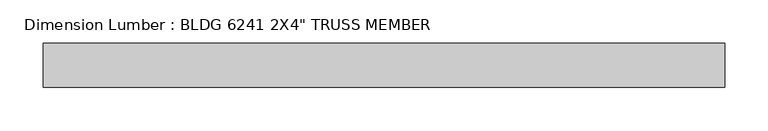
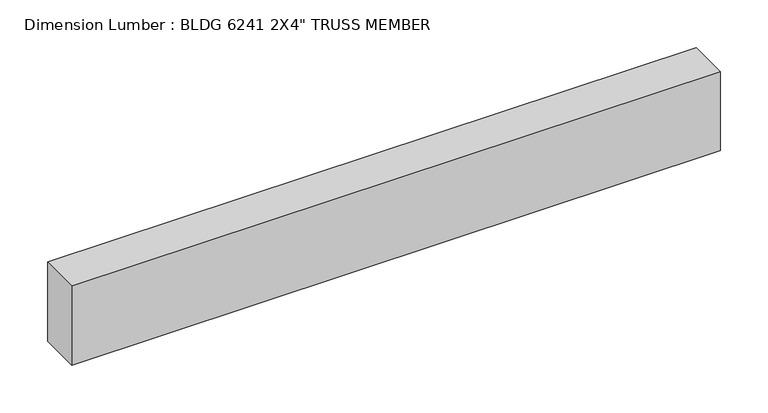
"""IFC4 building model written with IfcOpenShell, lengths in millimetres: beam geometry."""

from ifc_helpers import new_model, si_unit, frame, origin, place, context, project, spatial, polyline, outline, extrude, source, transform, mapped, element, save


def beam_f00f3f92(model_context):
    return source(origin(), model_context, "Body", "SweptSolid", [
        extrude(outline(polyline([(393.7, -25.4), (-393.7, -25.4), (-393.7, 25.4), (393.7, 25.4), (393.7, -25.4)])), frame((0.0, 0.0, -50.8), z_axis=(0.0, 0.0, 1.0), x_axis=(1.0, 0.0, 0.0)), (0.0, 0.0, 1.0), 101.6),
    ])


if __name__ == "__main__":
    model = new_model("IFC4")
    model_context = context("Model", 3, world=origin())
    ifc_project = project(units=[si_unit("LENGTHUNIT", "METRE", prefix="MILLI")], contexts=[model_context])
    site = spatial("IfcSite", under=ifc_project)
    building = spatial("IfcBuilding", under=site)
    placement = place(None, origin())
    beam_shape = beam_f00f3f92(model_context)
    element("IfcBeam", 1, ObjectType="Dimension Lumber : BLDG 6241 2X4\" TRUSS MEMBER", at=placement, inside=building, context=model_context, shape_type="MappedRepresentation", body=[
        mapped(beam_shape, transform((0.0, 0.0, 0.0), x_axis=(1.0, 0.0, 0.0), y_axis=(0.0, 1.0, 0.0), z_axis=(0.0, 0.0, 1.0))),
    ])
    save(model, "model.ifc")

# Revit data of these elements
# Type "Dimension Lumber : BLDG 6241 2X4\" TRUSS MEMBER"
#   Assembly Code = "B10"
#   A = 0.273472 SF
#   Length [instance default] = 5' - 0"
#   b = 0' - 2"
#   d = 0' - 4"
#   Structural Material [instance default] = Softwood, Lumber
# Element 1 (IfcBeam, "Dimension Lumber : BLDG 6241 2X4\" TRUSS MEMBER")
#   Materials on its faces: "Softwood, Lumber"
# Materials
#   "Softwood, Lumber": class "Wood", colour RGB 223 192 134, transparency 0, Description = "Pinus Echinata", Cost = 0
